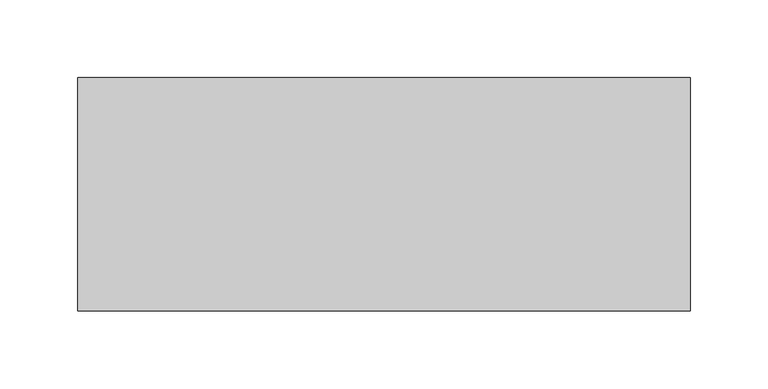
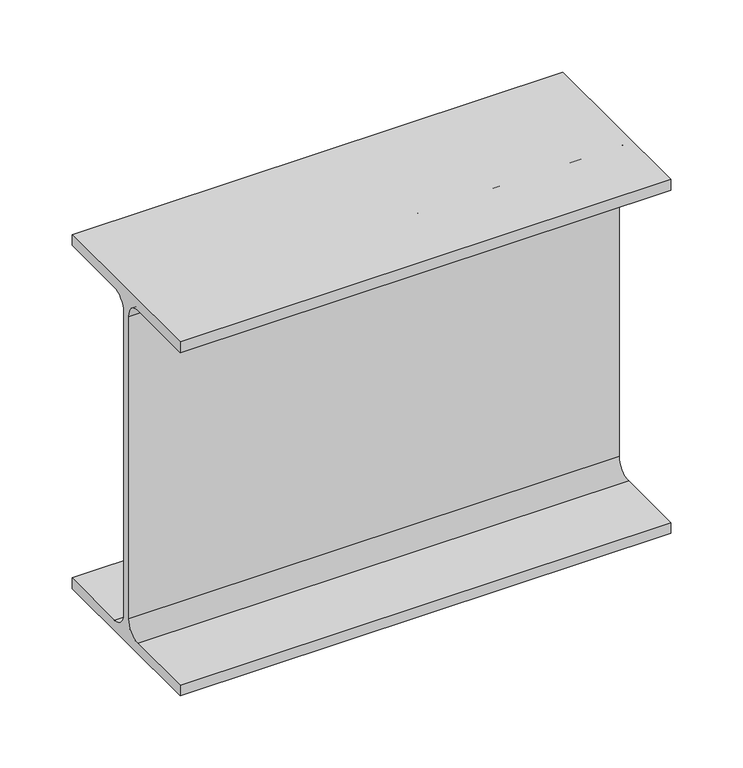
"""IFC4 building model written with IfcOpenShell, lengths in millimetres: beam geometry, 0912_Steel Framing_H-KSD3502 : H_SB_ASB_H-300x150x6.5x9."""

import ifcopenshell
import ifcopenshell.guid

model = None  # the IFC model being written
_history = None  # IfcOwnerHistory: only IFC2X3 demands one
_inside = {}  # id of a spatial element -> (the spatial element, [elements in it])
_under = {}  # id of a project, library or spatial element -> (it, [spatial elements below it])
_declared = {}  # id of a project -> (the project, [libraries it declares])
_typed = {}  # id of a type object -> (the type object, [elements of that type])
_made_of = {}  # id of a material, layer set ... -> (it, [elements and type objects made of it])


def new_model(schema):
    """Start an empty IFC model of exactly this schema.

    Asked for "IFC4X3", IfcOpenShell would pick the latest addendum, in which some entities
    have other attributes; the version numbers below select the first issue.
    IFC2X3 requires an IfcOwnerHistory on every rooted entity: one is made here for all.
    """
    global model, _history
    if schema == "IFC4X3":
        model = ifcopenshell.file(schema_version=(4, 3, 0, 0))
    else:
        model = ifcopenshell.file(schema=schema)
    _inside.clear()
    _under.clear()
    _declared.clear()
    _typed.clear()
    _made_of.clear()
    _history = None
    if model.schema == "IFC2X3":
        org = make("IfcOrganization", Name="unknown")
        user = make(
            "IfcPersonAndOrganization",
            ThePerson=make("IfcPerson", FamilyName="unknown"),
            TheOrganization=org,
        )
        app = make(
            "IfcApplication",
            ApplicationDeveloper=org,
            Version="unknown",
            ApplicationFullName="unknown",
            ApplicationIdentifier="unknown",
        )
        _history = make(
            "IfcOwnerHistory",
            OwningUser=user,
            OwningApplication=app,
            ChangeAction="ADDED",
            CreationDate=0,
        )
    return model


def make(cls, **values):
    """One entity of the class cls with the attributes given. An attribute that is None is left unset."""
    return model.create_entity(
        cls, **{name: value for name, value in values.items() if value is not None}
    )


def rooted(cls, **values):
    """An entity with a GlobalId (a new one), such as an element, a storey or a relation."""
    return make(cls, GlobalId=ifcopenshell.guid.new(), OwnerHistory=_history, **values)


def si_unit(unit_type, name, prefix=None):
    """IfcSIUnit, for example si_unit("LENGTHUNIT", "METRE", prefix="MILLI")."""
    return make("IfcSIUnit", UnitType=unit_type, Prefix=prefix, Name=name)


def assignment(units):
    """IfcUnitAssignment: the units of a project."""
    return None if units is None else make("IfcUnitAssignment", Units=units)


def point(xyz):
    """IfcCartesianPoint."""
    return None if xyz is None else make("IfcCartesianPoint", Coordinates=xyz)


def direction(xyz):
    """IfcDirection."""
    return None if xyz is None else make("IfcDirection", DirectionRatios=xyz)


def frame(location, z_axis=None, x_axis=None):
    """IfcAxis2Placement3D, a coordinate frame: its origin and axes. An axis left out is left unset."""
    return make(
        "IfcAxis2Placement3D",
        Location=point(location),
        Axis=direction(z_axis),
        RefDirection=direction(x_axis),
    )


def frame_2d(location, x_axis=None):
    """IfcAxis2Placement2D, a coordinate frame in the plane: its origin and x axis."""
    return make(
        "IfcAxis2Placement2D", Location=point(location), RefDirection=direction(x_axis)
    )


def origin():
    """The frame at (0, 0, 0) with its axes left unset."""
    return frame((0.0, 0.0, 0.0))


def place(relative_to, where):
    """IfcLocalPlacement: puts the frame where relative to a parent placement (None: the world)."""
    return make(
        "IfcLocalPlacement", PlacementRelTo=relative_to, RelativePlacement=where
    )


def context(
    kind, dimensions, precision=None, world=None, true_north=None, identifier=None
):
    """IfcGeometricRepresentationContext, for example the 3D "Model" context."""
    return make(
        "IfcGeometricRepresentationContext",
        ContextIdentifier=identifier,
        ContextType=kind,
        CoordinateSpaceDimension=dimensions,
        Precision=precision,
        WorldCoordinateSystem=world,
        TrueNorth=true_north,
    )


def project(units=None, contexts=None):
    """IfcProject with its units and contexts."""
    return rooted(
        "IfcProject",
        Name="project",
        RepresentationContexts=contexts,
        UnitsInContext=assignment(units),
    )


def spatial(cls, under=None, at=None, **own):
    """A site, building, storey or space (cls), placed at a placement, below another one or the project."""
    s = rooted(cls, ObjectPlacement=at, **own)
    if under is not None:
        _under.setdefault(under.id(), (under, []))[1].append(s)
    return s


def polyline(points):
    """IfcPolyline through the points."""
    return make("IfcPolyline", Points=[point(p) for p in points])


def circle_curve(where, radius):
    """IfcCircle in the frame where."""
    return make("IfcCircle", Position=where, Radius=radius)


def trimmed(basis, trim1, trim2, sense, master):
    """IfcTrimmedCurve: the piece of a basis curve between two trims."""
    return make(
        "IfcTrimmedCurve",
        BasisCurve=basis,
        Trim1=trim1,
        Trim2=trim2,
        SenseAgreement=sense,
        MasterRepresentation=master,
    )


def segment(curve, same_sense, transition):
    """IfcCompositeCurveSegment."""
    return make(
        "IfcCompositeCurveSegment",
        Transition=transition,
        SameSense=same_sense,
        ParentCurve=curve,
    )


def composite_curve(segments, self_intersect=None):
    """IfcCompositeCurve: segments joined end to end."""
    return make("IfcCompositeCurve", Segments=segments, SelfIntersect=self_intersect)


def outline(outer, holes=None, kind="AREA"):
    """IfcArbitraryClosedProfileDef: a profile drawn as a closed curve; with holes, ...WithVoids."""
    if holes is None:
        return make("IfcArbitraryClosedProfileDef", ProfileType=kind, OuterCurve=outer)
    return make(
        "IfcArbitraryProfileDefWithVoids",
        ProfileType=kind,
        OuterCurve=outer,
        InnerCurves=holes,
    )


def extrude(swept, where, along, depth):
    """IfcExtrudedAreaSolid: the profile swept, set in the frame where, extruded along a direction by depth."""
    return make(
        "IfcExtrudedAreaSolid",
        SweptArea=swept,
        Position=where,
        ExtrudedDirection=direction(along),
        Depth=depth,
    )


def shape(context_of_items, identifier, shape_type, items):
    """IfcShapeRepresentation: the items that make up one representation, for example the "Body"."""
    return make(
        "IfcShapeRepresentation",
        ContextOfItems=context_of_items,
        RepresentationIdentifier=identifier,
        RepresentationType=shape_type,
        Items=items,
    )


def source(mapping_origin, context_of_items, identifier, shape_type, items):
    """IfcRepresentationMap: a shape defined once, which mapped items show again and again."""
    return make(
        "IfcRepresentationMap",
        MappingOrigin=mapping_origin,
        MappedRepresentation=shape(context_of_items, identifier, shape_type, items),
    )


def transform(
    local_origin,
    x_axis=None,
    y_axis=None,
    z_axis=None,
    scale=None,
    scale2=None,
    scale3=None,
    uniform=True,
):
    """IfcCartesianTransformationOperator3D, or its non-uniform kind. x_axis, y_axis, z_axis: its Axis1, 2, 3."""
    if uniform:
        return make(
            "IfcCartesianTransformationOperator3D",
            Axis1=direction(x_axis),
            Axis2=direction(y_axis),
            LocalOrigin=point(local_origin),
            Scale=scale,
            Axis3=direction(z_axis),
        )
    return make(
        "IfcCartesianTransformationOperator3DnonUniform",
        Axis1=direction(x_axis),
        Axis2=direction(y_axis),
        LocalOrigin=point(local_origin),
        Scale=scale,
        Axis3=direction(z_axis),
        Scale2=scale2,
        Scale3=scale3,
    )


def mapped(mapping_source, mapping_target):
    """IfcMappedItem: shows the shape of a source again, moved by a transform."""
    return make(
        "IfcMappedItem", MappingSource=mapping_source, MappingTarget=mapping_target
    )


def made_of(thing, what):
    """Note that an element or type object is made of a material, layer set ...; save() writes the relation."""
    if what is not None:
        _made_of.setdefault(what.id(), (what, []))[1].append(thing)
    return thing


def element(
    cls,
    number,
    at=None,
    inside=None,
    cuts=None,
    type_object=None,
    material=None,
    context=None,
    identifier="Body",
    shape_type=None,
    held_by="IfcProductDefinitionShape",
    body=None,
    shapes=None,
    **own,
):
    """One element of the class cls, such as IfcWall. Its Tag is "e" and its number.

    at: its placement. inside: the storey or other place that contains it. cuts: it is an
    opening in that element (IfcRelVoidsElement). A single representation is given by context,
    identifier, shape_type and body (its items); several are given by shapes. held_by: the class
    of the entity that holds the representations. save() writes the other relations.
    """
    e = rooted(cls, Tag="e%d" % number, ObjectPlacement=at, **own)
    if body is not None:
        shapes = [shape(context, identifier, shape_type, body)]
    if shapes is not None:
        e.Representation = make(held_by, Representations=shapes)
    if inside is not None:
        _inside.setdefault(inside.id(), (inside, []))[1].append(e)
    if cuts is not None:
        rooted(
            "IfcRelVoidsElement", RelatingBuildingElement=cuts, RelatedOpeningElement=e
        )
    if type_object is not None:
        _typed.setdefault(type_object.id(), (type_object, []))[1].append(e)
    return made_of(e, material)


def aggregate(whole, parts):
    """IfcRelAggregates: a whole, such as a stair, and the parts it consists of."""
    return rooted("IfcRelAggregates", RelatingObject=whole, RelatedObjects=parts)


def save(model, path):
    """Write the relations noted so far, then the file.

    IfcRelAggregates (storeys below a building ...), IfcRelContainedInSpatialStructure (elements
    in a storey), IfcRelDefinesByType, IfcRelAssociatesMaterial and IfcRelDeclares: one each for
    every whole, place, type object, material and project.
    """
    for whole, parts in _under.values():
        aggregate(whole, parts)
    for where, things in _inside.values():
        rooted(
            "IfcRelContainedInSpatialStructure",
            RelatedElements=things,
            RelatingStructure=where,
        )
    for kind, things in _typed.values():
        rooted("IfcRelDefinesByType", RelatedObjects=things, RelatingType=kind)
    for what, things in _made_of.values():
        rooted("IfcRelAssociatesMaterial", RelatedObjects=things, RelatingMaterial=what)
    for by, libraries in _declared.values():
        rooted("IfcRelDeclares", RelatingContext=by, RelatedDefinitions=libraries)
    model.write(path)


def beam_3f731998(model_context):
    return source(origin(), model_context, "Body", "SweptSolid", [
        extrude(outline(composite_curve([segment(polyline([(75.0, -141.0), (75.0, -150.0), (-75.0, -150.0), (-75.0, -141.0), (-16.25, -141.0)]), True, "CONTINUOUS"), segment(trimmed(circle_curve(frame_2d((-16.25, -128.0)), 13.0), [point((-16.25, -141.0))], [point((-3.25, -128.0))], True, "CARTESIAN"), True, "CONTINUOUS"), segment(polyline([(-3.25, -128.0), (-3.25, 128.0)]), True, "CONTINUOUS"), segment(trimmed(circle_curve(frame_2d((-16.25, 128.0)), 13.0), [point((-3.25, 128.0))], [point((-16.25, 141.0))], True, "CARTESIAN"), True, "CONTINUOUS"), segment(polyline([(-16.25, 141.0), (-75.0, 141.0), (-75.0, 150.0), (75.0, 150.0), (75.0, 141.0), (16.25, 141.0)]), True, "CONTINUOUS"), segment(trimmed(circle_curve(frame_2d((16.25, 128.0)), 13.0), [point((16.25, 141.0))], [point((3.25, 128.0))], True, "CARTESIAN"), True, "CONTINUOUS"), segment(polyline([(3.25, 128.0), (3.25, -128.0)]), True, "CONTINUOUS"), segment(trimmed(circle_curve(frame_2d((16.25, -128.0)), 13.0), [point((3.25, -128.0))], [point((16.25, -141.0))], True, "CARTESIAN"), True, "CONTINUOUS"), segment(polyline([(16.25, -141.0), (75.0, -141.0)]), True, "CONTINUOUS")], self_intersect=False)), frame((-190.2999994, 0.0, 0.0), z_axis=(1.0, 0.0, 0.0), x_axis=(0.0, 1.0, 0.0)), (0.0, 0.0, 1.0), 393.2999994),
    ])


if __name__ == "__main__":
    model = new_model("IFC4")
    model_context = context("Model", 3, world=origin())
    ifc_project = project(units=[si_unit("LENGTHUNIT", "METRE", prefix="MILLI")], contexts=[model_context])
    site = spatial("IfcSite", under=ifc_project)
    building = spatial("IfcBuilding", under=site)
    placement = place(None, origin())
    beam_shape = beam_3f731998(model_context)
    element("IfcBeam", 1, ObjectType="0912_Steel Framing_H-KSD3502 : H_SB_ASB_H-300x150x6.5x9", at=placement, inside=building, context=model_context, shape_type="MappedRepresentation", body=[
        mapped(beam_shape, transform((0.0, 0.0, 0.0), x_axis=(1.0, 0.0, 0.0), y_axis=(0.0, 1.0, 0.0), z_axis=(0.0, 0.0, 1.0))),
    ])
    save(model, "model.ifc")

# Revit data of these elements
# Type "0912_Steel Framing_H-KSD3502 : H_SB_ASB_H-300x150x6.5x9"
#   H_WM Code_1 = "S01AA002-00001 | Main Steel Structure Fabrication Work | Shelter/Building | Medium Steel - Standard (90KG/M>Weight≥30KG/M) | Material: (   )"
#   H_WM Code_2 = "S03AA028-00001 | Main Steel Structure Erection Work | Shelter/Building | Medium Steel (90KG/M>Weight≥30KG/M) | Material: (   )"
#   H_WM Code_3 = "S01AA010-00001 | Main Steel Structure Fabrication Work | Shelter/Building | Steel Painting/Coating | for Non-Fireproofed Steel Surface, Surface Preparation, Primer, Second & Final Coat | Material: (   )"
#   H_Q'ty Cal Type Tag = "SB-Q2"
#   Width = 15.0 cm
#   Web Thickness = 0.65 cm
#   Web Fillet = 1.3 cm
#   Warping Constant = 107000.0 cm⁶
#   W = 0
#   Torsional Moment of Inertia = 9.9539 cm⁴
#   Section Area = 46.78 cm²
#   Plastic Modulus weak axis = 105.0 cm³
#   Plastic Modulus strong axis = 542.0 cm³
#   Perimeter = 1.17 m²/m
#   Nominal Weight = 36.70 kgf/m
#   Moment of Inertia weak axis = 508.00 cm⁴
#   Moment of Inertia strong axis = 7210.00 cm⁴
#   Height = 30.0 cm
#   Flange Thickness = 0.9 cm
#   Elastic Modulus weak axis = 67.7 cm³
#   Elastic Modulus strong axis = 481.0 cm³
#   Centroid Vertical = 15.0 cm
#   Centroid Horizontal = 7.5 cm
#   Ix = 72100000
#   Length [instance default] = 1.5240 m
#   Zx = 542000
#   b = 0.1500 m
#   h = 0.3000 m
#   r = 0.0130 m
#   s = 0.0065 m
#   t = 0.0090 m
#   A = 0.004678 m²
#   Structural Material [instance default] = Steel, 45-345
#   Assembly Code = ""
# Element 1 (IfcBeam, "0912_Steel Framing_H-KSD3502 : H_SB_ASB_H-300x150x6.5x9")
#   Structural Material = none
# Materials
#   "Steel, 45-345": class "Metal", colour RGB 189 187 185, transparency 0, Description = "Steel 345 MPa", Cost = 0
